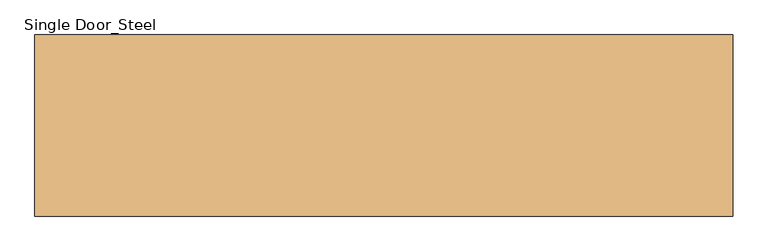
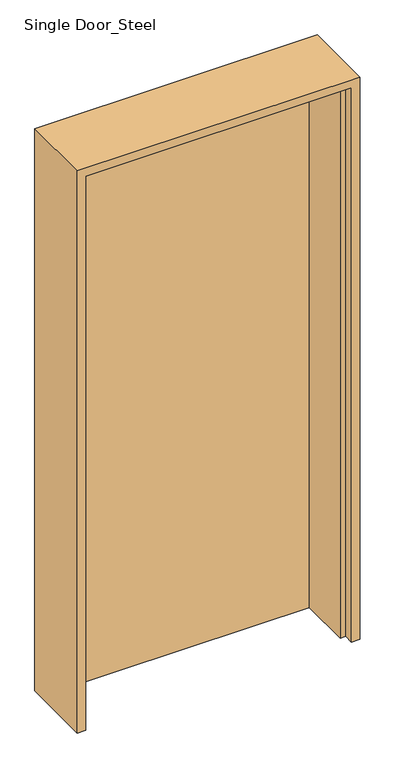
"""IFC4 building model written with IfcOpenShell, lengths in millimetres: door geometry, Single Door_Steel : H_DR_AR_B12_Single Door_Steel_W1000xH2100."""

from ifc_helpers import new_model, si_unit, origin, origin_with_axes, place, context, project, spatial, polyline, outline, extrude, faceted_brep, source, transform, mapped, element, save


def single_door_steel_4a6c7de9(model_context):
    return source(origin(), model_context, "Body", "SolidModel", [
        extrude(outline(polyline([(470.0, 130.0), (470.0, 95.0), (-470.0, 95.0), (-470.0, 130.0), (470.0, 130.0)])), origin_with_axes(), (0.0, 0.0, 1.0), 2070.0),
        faceted_brep([(470.0, 130.0, 0.0), (500.0, 130.0, 0.0), (500.0, -130.0, 0.0), (470.0, -130.0, 0.0), (470.0, -95.0, 0.0), (450.0, -95.0, 0.0), (450.0, 95.0, 0.0), (470.0, 95.0, 0.0), (470.0, 130.0, 2070.0), (-470.0, 130.0, 2070.0), (-470.0, 130.0, 0.0), (-500.0, 130.0, 0.0), (-500.0, 130.0, 2100.0), (500.0, 130.0, 2100.0), (500.0, -130.0, 2100.0), (-500.0, -130.0, 2100.0), (-500.0, -130.0, 0.0), (-470.0, -130.0, 0.0), (-470.0, -130.0, 2070.0), (470.0, -130.0, 2070.0), (470.0, -95.0, 2070.0), (-470.0, -95.0, 2070.0), (-470.0, -95.0, 0.0), (-450.0, -95.0, 0.0), (-450.0, -95.0, 2050.0), (450.0, -95.0, 2050.0), (450.0, 95.0, 2050.0), (-450.0, 95.0, 2050.0), (-450.0, 95.0, 0.0), (-470.0, 95.0, 0.0), (-470.0, 95.0, 2070.0), (470.0, 95.0, 2070.0)], [[[0, 1, 2, 3, 4, 5, 6, 7]], [[1, 0, 8, 9, 10, 11, 12, 13]], [[2, 1, 13, 14]], [[3, 2, 14, 15, 16, 17, 18, 19]], [[4, 3, 19, 20]], [[5, 4, 20, 21, 22, 23, 24, 25]], [[6, 5, 25, 26]], [[7, 6, 26, 27, 28, 29, 30, 31]], [[0, 7, 31, 8]], [[9, 30, 29, 10]], [[10, 29, 28, 23, 22, 17, 16, 11]], [[15, 12, 11, 16]], [[21, 18, 17, 22]], [[27, 24, 23, 28]], [[14, 13, 12, 15]], [[20, 19, 18, 21]], [[26, 25, 24, 27]], [[8, 31, 30, 9]]]),
    ])


if __name__ == "__main__":
    model = new_model("IFC4")
    model_context = context("Model", 3, world=origin())
    ifc_project = project(units=[si_unit("LENGTHUNIT", "METRE", prefix="MILLI")], contexts=[model_context])
    site = spatial("IfcSite", under=ifc_project)
    building = spatial("IfcBuilding", under=site)
    placement = place(None, origin())
    single_door_steel_shape = single_door_steel_4a6c7de9(model_context)
    element("IfcDoor", 1, ObjectType="Single Door_Steel : H_DR_AR_B12_Single Door_Steel_W1000xH2100", at=placement, inside=building, context=model_context, shape_type="MappedRepresentation", body=[
        mapped(single_door_steel_shape, transform((0.0, 0.0, 0.0), x_axis=(1.0, 0.0, 0.0), y_axis=(0.0, 1.0, 0.0), z_axis=(0.0, 0.0, 1.0))),
    ])
    save(model, "model.ifc")

# Revit data of these elements
# Type "Single Door_Steel : H_DR_AR_B12_Single Door_Steel_W1000xH2100"
#   Type Mark = "SD"
#   Analytic Construction = "<None>"
#   프레임 투영 외부. = 25 mm
#   프레임 투영 내부. = 25 mm
#   프레임 폭 = 75 mm
#   Height = 2100 mm
#   Width = 1000 mm
#   Define Thermal Properties by = 1
#   문 패널 = none
#   문 프레임 = none
#   Function = (empty or 0)
#   Wall Closure = (empty or 0)
